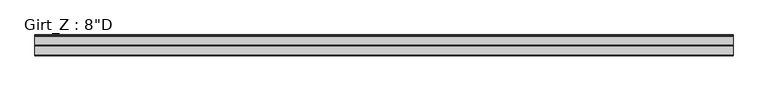
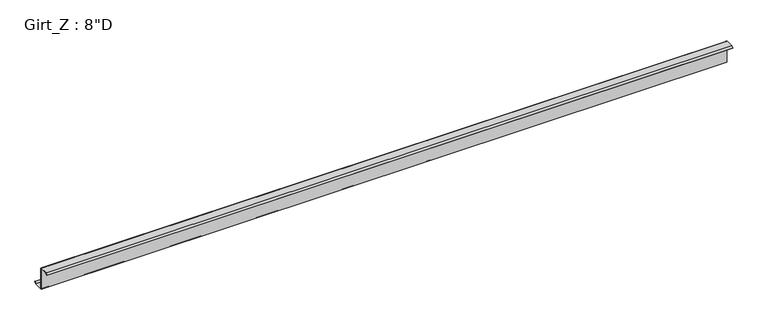
"""IFC4 building model written with IfcOpenShell, lengths in millimetres: beam geometry."""

from ifc_helpers import new_model, si_unit, point, frame, frame_2d, origin, place, context, project, spatial, polyline, circle_curve, trimmed, segment, composite_curve, outline, extrude, source, transform, mapped, element, save


def beam_ab2f8a8d(model_context):
    return source(origin(), model_context, "Body", "SweptSolid", [
        extrude(outline(composite_curve([segment(polyline([(-77.9859375, 101.6), (-3.3734375, 101.6)]), True, "CONTINUOUS"), segment(trimmed(circle_curve(frame_2d((-3.3734375, 96.8375)), 4.7625), [point((-3.3734375, 101.6))], [point((1.3890625, 96.8375))], False, "CARTESIAN"), True, "CONTINUOUS"), segment(polyline([(1.3890625, 96.8375), (1.3890625, -96.8389339)]), True, "CONTINUOUS"), segment(trimmed(circle_curve(frame_2d((3.3748024, -96.8389339)), 1.9857399), [point((1.3890625, -96.8389339))], [point((3.2694106, -98.821875))], True, "CARTESIAN"), True, "CONTINUOUS"), segment(polyline([(3.2694106, -98.821875), (83.0404765, -98.821875), (94.4528742, -85.221109), (96.5810415, -87.0068534), (84.3359375, -101.6), (-1.3890625, -101.6), (-1.3890625, 96.8381931)]), True, "CONTINUOUS"), segment(trimmed(circle_curve(frame_2d((-3.3741066, 96.8381931)), 1.9850441), [point((-1.3890625, 96.8381931))], [point((-3.3005807, 98.821875))], True, "CARTESIAN"), True, "CONTINUOUS"), segment(polyline([(-3.3005807, 98.821875), (-76.6904765, 98.821875), (-88.1028742, 85.221109), (-90.2310415, 87.0068534), (-77.9859375, 101.6)]), True, "CONTINUOUS")], self_intersect=False)), frame((-3100.3875, 0.0, 0.0), z_axis=(1.0, 0.0, 0.0), x_axis=(0.0, 1.0, 0.0)), (0.0, 0.0, 1.0), 6200.775),
    ])


if __name__ == "__main__":
    model = new_model("IFC4")
    model_context = context("Model", 3, world=origin())
    ifc_project = project(units=[si_unit("LENGTHUNIT", "METRE", prefix="MILLI")], contexts=[model_context])
    site = spatial("IfcSite", under=ifc_project)
    building = spatial("IfcBuilding", under=site)
    placement = place(None, origin())
    beam_shape = beam_ab2f8a8d(model_context)
    element("IfcBeam", 1, ObjectType="Girt_Z : 8\"D", at=placement, inside=building, context=model_context, shape_type="MappedRepresentation", body=[
        mapped(beam_shape, transform((0.0, 0.0, 0.0), x_axis=(1.0, 0.0, 0.0), y_axis=(0.0, 1.0, 0.0), z_axis=(0.0, 0.0, 1.0))),
    ])
    save(model, "model.ifc")

# Revit data of these elements
# Type "Girt_Z : 8\"D"
#   half leg = 0' - 1 11/16"
#   Web_Thickness = 0' - 0 7/64"
#   Length [instance default] = 10' - 0"
#   Leg_2 = 0' - 3 3/8"
#   Leg_1 = 0' - 3 1/8"
#   Height = 0' - 8"
#   Structural Material [instance default] = none
